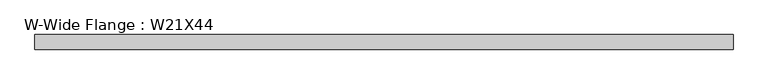
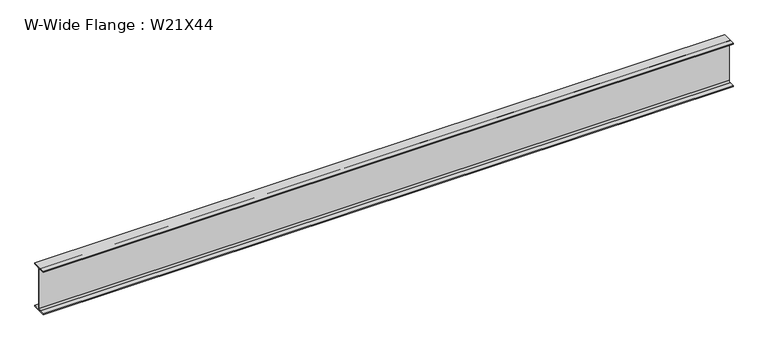
"""IFC4 building model written with IfcOpenShell, lengths in millimetres: beam geometry, W-Wide Flange : W21X44."""

import ifcopenshell
import ifcopenshell.guid

model = None  # the IFC model being written
_history = None  # IfcOwnerHistory: only IFC2X3 demands one
_inside = {}  # id of a spatial element -> (the spatial element, [elements in it])
_under = {}  # id of a project, library or spatial element -> (it, [spatial elements below it])
_declared = {}  # id of a project -> (the project, [libraries it declares])
_typed = {}  # id of a type object -> (the type object, [elements of that type])
_made_of = {}  # id of a material, layer set ... -> (it, [elements and type objects made of it])


def new_model(schema):
    """Start an empty IFC model of exactly this schema.

    Asked for "IFC4X3", IfcOpenShell would pick the latest addendum, in which some entities
    have other attributes; the version numbers below select the first issue.
    IFC2X3 requires an IfcOwnerHistory on every rooted entity: one is made here for all.
    """
    global model, _history
    if schema == "IFC4X3":
        model = ifcopenshell.file(schema_version=(4, 3, 0, 0))
    else:
        model = ifcopenshell.file(schema=schema)
    _inside.clear()
    _under.clear()
    _declared.clear()
    _typed.clear()
    _made_of.clear()
    _history = None
    if model.schema == "IFC2X3":
        org = make("IfcOrganization", Name="unknown")
        user = make(
            "IfcPersonAndOrganization",
            ThePerson=make("IfcPerson", FamilyName="unknown"),
            TheOrganization=org,
        )
        app = make(
            "IfcApplication",
            ApplicationDeveloper=org,
            Version="unknown",
            ApplicationFullName="unknown",
            ApplicationIdentifier="unknown",
        )
        _history = make(
            "IfcOwnerHistory",
            OwningUser=user,
            OwningApplication=app,
            ChangeAction="ADDED",
            CreationDate=0,
        )
    return model


def make(cls, **values):
    """One entity of the class cls with the attributes given. An attribute that is None is left unset."""
    return model.create_entity(
        cls, **{name: value for name, value in values.items() if value is not None}
    )


def rooted(cls, **values):
    """An entity with a GlobalId (a new one), such as an element, a storey or a relation."""
    return make(cls, GlobalId=ifcopenshell.guid.new(), OwnerHistory=_history, **values)


def si_unit(unit_type, name, prefix=None):
    """IfcSIUnit, for example si_unit("LENGTHUNIT", "METRE", prefix="MILLI")."""
    return make("IfcSIUnit", UnitType=unit_type, Prefix=prefix, Name=name)


def assignment(units):
    """IfcUnitAssignment: the units of a project."""
    return None if units is None else make("IfcUnitAssignment", Units=units)


def point(xyz):
    """IfcCartesianPoint."""
    return None if xyz is None else make("IfcCartesianPoint", Coordinates=xyz)


def direction(xyz):
    """IfcDirection."""
    return None if xyz is None else make("IfcDirection", DirectionRatios=xyz)


def frame(location, z_axis=None, x_axis=None):
    """IfcAxis2Placement3D, a coordinate frame: its origin and axes. An axis left out is left unset."""
    return make(
        "IfcAxis2Placement3D",
        Location=point(location),
        Axis=direction(z_axis),
        RefDirection=direction(x_axis),
    )


def frame_2d(location, x_axis=None):
    """IfcAxis2Placement2D, a coordinate frame in the plane: its origin and x axis."""
    return make(
        "IfcAxis2Placement2D", Location=point(location), RefDirection=direction(x_axis)
    )


def origin():
    """The frame at (0, 0, 0) with its axes left unset."""
    return frame((0.0, 0.0, 0.0))


def place(relative_to, where):
    """IfcLocalPlacement: puts the frame where relative to a parent placement (None: the world)."""
    return make(
        "IfcLocalPlacement", PlacementRelTo=relative_to, RelativePlacement=where
    )


def context(
    kind, dimensions, precision=None, world=None, true_north=None, identifier=None
):
    """IfcGeometricRepresentationContext, for example the 3D "Model" context."""
    return make(
        "IfcGeometricRepresentationContext",
        ContextIdentifier=identifier,
        ContextType=kind,
        CoordinateSpaceDimension=dimensions,
        Precision=precision,
        WorldCoordinateSystem=world,
        TrueNorth=true_north,
    )


def project(units=None, contexts=None):
    """IfcProject with its units and contexts."""
    return rooted(
        "IfcProject",
        Name="project",
        RepresentationContexts=contexts,
        UnitsInContext=assignment(units),
    )


def spatial(cls, under=None, at=None, **own):
    """A site, building, storey or space (cls), placed at a placement, below another one or the project."""
    s = rooted(cls, ObjectPlacement=at, **own)
    if under is not None:
        _under.setdefault(under.id(), (under, []))[1].append(s)
    return s


def polyline(points):
    """IfcPolyline through the points."""
    return make("IfcPolyline", Points=[point(p) for p in points])


def circle_curve(where, radius):
    """IfcCircle in the frame where."""
    return make("IfcCircle", Position=where, Radius=radius)


def trimmed(basis, trim1, trim2, sense, master):
    """IfcTrimmedCurve: the piece of a basis curve between two trims."""
    return make(
        "IfcTrimmedCurve",
        BasisCurve=basis,
        Trim1=trim1,
        Trim2=trim2,
        SenseAgreement=sense,
        MasterRepresentation=master,
    )


def segment(curve, same_sense, transition):
    """IfcCompositeCurveSegment."""
    return make(
        "IfcCompositeCurveSegment",
        Transition=transition,
        SameSense=same_sense,
        ParentCurve=curve,
    )


def composite_curve(segments, self_intersect=None):
    """IfcCompositeCurve: segments joined end to end."""
    return make("IfcCompositeCurve", Segments=segments, SelfIntersect=self_intersect)


def outline(outer, holes=None, kind="AREA"):
    """IfcArbitraryClosedProfileDef: a profile drawn as a closed curve; with holes, ...WithVoids."""
    if holes is None:
        return make("IfcArbitraryClosedProfileDef", ProfileType=kind, OuterCurve=outer)
    return make(
        "IfcArbitraryProfileDefWithVoids",
        ProfileType=kind,
        OuterCurve=outer,
        InnerCurves=holes,
    )


def extrude(swept, where, along, depth):
    """IfcExtrudedAreaSolid: the profile swept, set in the frame where, extruded along a direction by depth."""
    return make(
        "IfcExtrudedAreaSolid",
        SweptArea=swept,
        Position=where,
        ExtrudedDirection=direction(along),
        Depth=depth,
    )


def shape(context_of_items, identifier, shape_type, items):
    """IfcShapeRepresentation: the items that make up one representation, for example the "Body"."""
    return make(
        "IfcShapeRepresentation",
        ContextOfItems=context_of_items,
        RepresentationIdentifier=identifier,
        RepresentationType=shape_type,
        Items=items,
    )


def source(mapping_origin, context_of_items, identifier, shape_type, items):
    """IfcRepresentationMap: a shape defined once, which mapped items show again and again."""
    return make(
        "IfcRepresentationMap",
        MappingOrigin=mapping_origin,
        MappedRepresentation=shape(context_of_items, identifier, shape_type, items),
    )


def transform(
    local_origin,
    x_axis=None,
    y_axis=None,
    z_axis=None,
    scale=None,
    scale2=None,
    scale3=None,
    uniform=True,
):
    """IfcCartesianTransformationOperator3D, or its non-uniform kind. x_axis, y_axis, z_axis: its Axis1, 2, 3."""
    if uniform:
        return make(
            "IfcCartesianTransformationOperator3D",
            Axis1=direction(x_axis),
            Axis2=direction(y_axis),
            LocalOrigin=point(local_origin),
            Scale=scale,
            Axis3=direction(z_axis),
        )
    return make(
        "IfcCartesianTransformationOperator3DnonUniform",
        Axis1=direction(x_axis),
        Axis2=direction(y_axis),
        LocalOrigin=point(local_origin),
        Scale=scale,
        Axis3=direction(z_axis),
        Scale2=scale2,
        Scale3=scale3,
    )


def mapped(mapping_source, mapping_target):
    """IfcMappedItem: shows the shape of a source again, moved by a transform."""
    return make(
        "IfcMappedItem", MappingSource=mapping_source, MappingTarget=mapping_target
    )


def made_of(thing, what):
    """Note that an element or type object is made of a material, layer set ...; save() writes the relation."""
    if what is not None:
        _made_of.setdefault(what.id(), (what, []))[1].append(thing)
    return thing


def element(
    cls,
    number,
    at=None,
    inside=None,
    cuts=None,
    type_object=None,
    material=None,
    context=None,
    identifier="Body",
    shape_type=None,
    held_by="IfcProductDefinitionShape",
    body=None,
    shapes=None,
    **own,
):
    """One element of the class cls, such as IfcWall. Its Tag is "e" and its number.

    at: its placement. inside: the storey or other place that contains it. cuts: it is an
    opening in that element (IfcRelVoidsElement). A single representation is given by context,
    identifier, shape_type and body (its items); several are given by shapes. held_by: the class
    of the entity that holds the representations. save() writes the other relations.
    """
    e = rooted(cls, Tag="e%d" % number, ObjectPlacement=at, **own)
    if body is not None:
        shapes = [shape(context, identifier, shape_type, body)]
    if shapes is not None:
        e.Representation = make(held_by, Representations=shapes)
    if inside is not None:
        _inside.setdefault(inside.id(), (inside, []))[1].append(e)
    if cuts is not None:
        rooted(
            "IfcRelVoidsElement", RelatingBuildingElement=cuts, RelatedOpeningElement=e
        )
    if type_object is not None:
        _typed.setdefault(type_object.id(), (type_object, []))[1].append(e)
    return made_of(e, material)


def aggregate(whole, parts):
    """IfcRelAggregates: a whole, such as a stair, and the parts it consists of."""
    return rooted("IfcRelAggregates", RelatingObject=whole, RelatedObjects=parts)


def save(model, path):
    """Write the relations noted so far, then the file.

    IfcRelAggregates (storeys below a building ...), IfcRelContainedInSpatialStructure (elements
    in a storey), IfcRelDefinesByType, IfcRelAssociatesMaterial and IfcRelDeclares: one each for
    every whole, place, type object, material and project.
    """
    for whole, parts in _under.values():
        aggregate(whole, parts)
    for where, things in _inside.values():
        rooted(
            "IfcRelContainedInSpatialStructure",
            RelatedElements=things,
            RelatingStructure=where,
        )
    for kind, things in _typed.values():
        rooted("IfcRelDefinesByType", RelatedObjects=things, RelatingType=kind)
    for what, things in _made_of.values():
        rooted("IfcRelAssociatesMaterial", RelatedObjects=things, RelatingMaterial=what)
    for by, libraries in _declared.values():
        rooted("IfcRelDeclares", RelatingContext=by, RelatedDefinitions=libraries)
    model.write(path)


def w_wide_flange_w21x44_8a3b57d7(model_context):
    return source(origin(), model_context, "Body", "SweptSolid", [
        extrude(outline(composite_curve([segment(polyline([(82.55, -251.46), (82.55, -262.89), (-82.55, -262.89), (-82.55, -251.46), (-21.59, -251.46)]), True, "CONTINUOUS"), segment(trimmed(circle_curve(frame_2d((-21.59, -234.315)), 17.145), [point((-21.59, -251.46))], [point((-4.445, -234.315))], True, "CARTESIAN"), True, "CONTINUOUS"), segment(polyline([(-4.445, -234.315), (-4.445, 234.315)]), True, "CONTINUOUS"), segment(trimmed(circle_curve(frame_2d((-21.59, 234.315)), 17.145), [point((-4.445, 234.315))], [point((-21.59, 251.46))], True, "CARTESIAN"), True, "CONTINUOUS"), segment(polyline([(-21.59, 251.46), (-82.55, 251.46), (-82.55, 262.89), (82.55, 262.89), (82.55, 251.46), (21.59, 251.46)]), True, "CONTINUOUS"), segment(trimmed(circle_curve(frame_2d((21.59, 234.315)), 17.145), [point((21.59, 251.46))], [point((4.445, 234.315))], True, "CARTESIAN"), True, "CONTINUOUS"), segment(polyline([(4.445, 234.315), (4.445, -234.315)]), True, "CONTINUOUS"), segment(trimmed(circle_curve(frame_2d((21.59, -234.315)), 17.145), [point((4.445, -234.315))], [point((21.59, -251.46))], True, "CARTESIAN"), True, "CONTINUOUS"), segment(polyline([(21.59, -251.46), (82.55, -251.46)]), True, "CONTINUOUS")], self_intersect=False)), frame((-3906.3890318, 0.0, 0.0), z_axis=(1.0, 0.0, 0.0), x_axis=(0.0, 1.0, 0.0)), (0.0, 0.0, 1.0), 7873.3579698),
    ])


if __name__ == "__main__":
    model = new_model("IFC4")
    model_context = context("Model", 3, world=origin())
    ifc_project = project(units=[si_unit("LENGTHUNIT", "METRE", prefix="MILLI")], contexts=[model_context])
    site = spatial("IfcSite", under=ifc_project)
    building = spatial("IfcBuilding", under=site)
    placement = place(None, origin())
    w_wide_flange_w21x44_shape = w_wide_flange_w21x44_8a3b57d7(model_context)
    element("IfcBeam", 1, ObjectType="W-Wide Flange : W21X44", at=placement, inside=building, context=model_context, shape_type="MappedRepresentation", body=[
        mapped(w_wide_flange_w21x44_shape, transform((0.0, 0.0, 0.0), x_axis=(1.0, 0.0, 0.0), y_axis=(0.0, 1.0, 0.0), z_axis=(0.0, 0.0, 1.0))),
    ])
    save(model, "model.ifc")

# Revit data of these elements
# Type "W-Wide Flange : W21X44"
#   Assembly Code = "B10"
#   W = 44
#   Length [instance default] = 1524 mm
#   bf = 165.1 mm
#   d = 525.78 mm
#   k = 28.575 mm
#   k2 = 17.145 mm
#   tf = 11.43 mm
#   tw = 8.89 mm
#   A = 0.00838708 m²
#   Structural Material [instance default] = Steel ASTM A992
# Element 1 (IfcBeam, "W-Wide Flange : W21X44")
#   Structural Material = Aluminum, Anodized Red
#   Materials on its faces: "Aluminum, Anodized Red"
# Materials
#   "Steel ASTM A992": class "Metal", colour RGB 128 0 0, transparency 0, Description = "Structural steel 50ksi", Cost = 0
#   "Aluminum, Anodized Red": class "Metal", colour RGB 120 120 120, transparency 0, Description = "Anodized aluminum, red", Cost = 0
